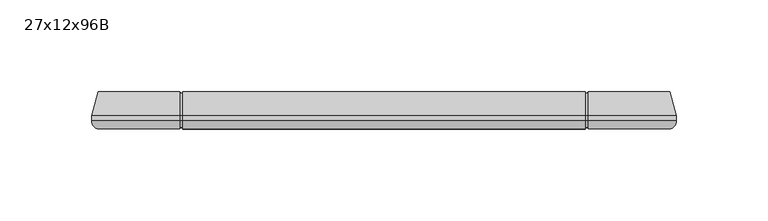
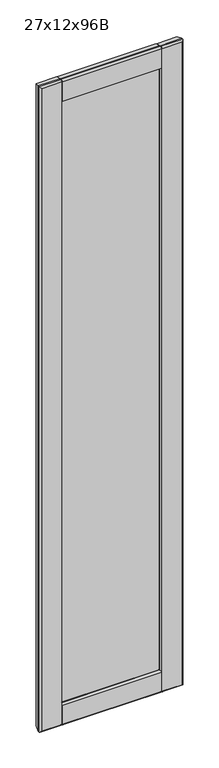
"""IFC4 building model written with IfcOpenShell, lengths in millimetres: furniture geometry, Cabinet-Tall-Merillat-Utility_Double-Marlin : 27x12x96B."""

from ifc_helpers import new_model, si_unit, frame, origin, place, context, project, spatial, polyline, circle_curve, ellipse_curve, outline, extrude, source, transform, mapped, element, save
from ifc_brep_helpers import plane_surface, cylinder_surface, advanced_brep


def furniture_27x12x96b_5ba57cf1(model_context):
    return source(origin(), model_context, "Body", "SolidModel", [
        advanced_brep(
        [(314.6646592, -320.6496, 1651.0), (311.5681667, -325.12, 1647.9035075), (311.5681667, -325.12, 142.7964925), (314.6646592, -320.6496, 139.7), (314.6646592, -317.881, 139.7), (314.6646592, -317.881, 1651.0), (311.1594592, -304.8, 143.2052), (311.1594592, -304.8, 1647.4948), (266.4634964, -304.8, 1602.7988372), (266.4634964, -304.8, 187.9011628), (266.0933647, -305.59375, 188.2712945), (264.0122057, -310.05681, 190.3524535), (264.0122057, -310.05681, 1600.3475465), (266.0933647, -305.59375, 1602.4287055), (265.4119751, -312.2969093, 188.952684), (265.4119751, -312.2969093, 1601.747316), (279.7396592, -312.547, 174.625), (279.7396592, -312.547, 1616.075), (279.7396592, -317.373, 174.625), (279.7396592, -317.373, 1616.075), (265.4119751, -317.6230907, 188.952684), (265.4119751, -317.6230907, 1601.747316), (264.0122057, -319.86319, 190.3524535), (264.0122057, -319.86319, 1600.3475465), (266.0933647, -324.32625, 188.2712945), (266.460629, -325.1138508, 187.9040302), (266.4634964, -325.12, 1602.7988372), (266.0933647, -324.32625, 1602.4287055), (266.460629, -325.12, 142.7964925), (266.460629, -320.6496, 139.7), (-1.3263483, -325.12, 142.7964925), (-4.4228408, -320.6496, 139.7), (43.7413778, -320.6496, 139.7), (43.7413778, -325.12, 142.7964925), (264.873129, -320.6496, 139.7), (264.873129, -325.12, 142.7964925), (45.3288778, -325.12, 142.7964925), (45.3288778, -320.6496, 139.7), (266.460629, -317.881, 139.7), (-4.4228408, -317.881, 139.7), (43.7413778, -317.881, 139.7), (264.873129, -317.881, 139.7), (45.3288778, -317.881, 139.7), (266.460629, -304.8, 143.2052), (-0.9176408, -304.8, 143.2052), (43.7413778, -304.8, 143.2052), (264.873129, -304.8, 143.2052), (45.3288778, -304.8, 143.2052), (46.2296127, -310.05681, 190.3524535), (264.873129, -305.59375, 188.2712945), (264.873129, -304.8, 187.9011628), (45.3288778, -304.8, 187.9011628), (45.3288778, -305.59375, 188.2712945), (44.1484536, -305.59375, 188.2712945), (44.8298432, -312.2969093, 188.952684), (30.5021592, -312.547, 174.625), (30.5021592, -317.373, 174.625), (44.8298432, -317.6230907, 188.952684), (46.2296127, -319.86319, 190.3524535), (44.1484536, -324.32625, 188.2712945), (45.3288778, -324.32625, 188.2712945), (45.3288778, -325.12, 187.9011628), (264.873129, -325.12, 187.9011628), (264.873129, -324.32625, 188.2712945), (-1.3263483, -325.12, 1647.9035075), (-4.4228408, -320.6496, 1651.0), (-4.4228408, -317.881, 1651.0), (-0.9176408, -304.8, 1647.4948), (43.7783219, -304.8, 187.9011628), (43.7783219, -304.8, 1602.7988372), (44.1484536, -305.59375, 1602.4287055), (46.2296127, -310.05681, 1600.3475465), (44.8298432, -312.2969093, 1601.747316), (30.5021592, -312.547, 1616.075), (30.5021592, -317.373, 1616.075), (44.8298432, -317.6230907, 1601.747316), (46.2296127, -319.86319, 1600.3475465), (44.1484536, -324.32625, 1602.4287055), (43.7783219, -325.12, 1602.7988372), (43.7783219, -325.12, 187.9011628), (43.7413778, -325.12, 1647.9035075), (43.7413778, -320.6496, 1651.0), (266.460629, -320.6496, 1651.0), (266.460629, -325.12, 1647.9035075), (45.3288778, -320.6496, 1651.0), (45.3288778, -325.12, 1647.9035075), (264.873129, -325.12, 1647.9035075), (264.873129, -320.6496, 1651.0), (43.7413778, -317.881, 1651.0), (266.460629, -317.881, 1651.0), (45.3288778, -317.881, 1651.0), (264.873129, -317.881, 1651.0), (43.7413778, -304.8, 1647.4948), (266.460629, -304.8, 1647.4948), (45.3288778, -304.8, 1647.4948), (264.873129, -304.8, 1647.4948), (45.3288778, -304.8, 1602.7988372), (264.873129, -304.8, 1602.7988372), (45.3288778, -305.59375, 1602.4287055), (264.873129, -305.59375, 1602.4287055), (264.873129, -324.32625, 1602.4287055), (264.873129, -325.12, 1602.7988372), (45.3288778, -325.12, 1602.7988372), (45.3288778, -324.32625, 1602.4287055), (45.3288778, -305.59375, 1646.8857412), (45.3288778, -317.9855037, 1650.20625), (45.3288778, -320.6496, 1650.20625), (45.3288778, -324.32625, 1647.7526052), (43.7413778, -324.32625, 1602.4287055), (43.7413778, -324.32625, 1647.7526052), (43.7413778, -320.6496, 1650.20625), (43.7413778, -317.9855037, 1650.20625), (43.7413778, -305.59375, 1646.8857412), (43.7413778, -305.59375, 1602.4287055), (266.460629, -305.59375, 1602.4287055), (266.460629, -305.59375, 1646.8857412), (266.460629, -317.9855037, 1650.20625), (266.460629, -320.6496, 1650.20625), (266.460629, -324.32625, 1647.7526052), (266.460629, -324.32625, 1602.4287055), (264.873129, -324.32625, 1647.7526052), (264.873129, -320.6496, 1650.20625), (264.873129, -317.9855037, 1650.20625), (264.873129, -305.59375, 1646.8857412), (266.460629, -324.32625, 188.2712945), (266.460629, -324.32625, 142.9473948), (266.460629, -320.6496, 140.49375), (266.460629, -317.9855037, 140.49375), (266.460629, -305.59375, 143.8142588), (266.460629, -305.59375, 188.2712945), (264.873129, -305.59375, 143.8142588), (264.873129, -317.9855037, 140.49375), (264.873129, -320.6496, 140.49375), (264.873129, -324.32625, 142.9473948), (45.3288778, -324.32625, 142.9473948), (45.3288778, -320.6496, 140.49375), (45.3288778, -317.9855037, 140.49375), (45.3288778, -305.59375, 143.8142588), (43.7413778, -324.32625, 188.2712945), (43.7413778, -305.59375, 188.2712945), (43.7413778, -305.59375, 143.8142588), (43.7413778, -317.9855037, 140.49375), (43.7413778, -320.6496, 140.49375), (43.7413778, -324.32625, 142.9473948)],
        [
            (0, 1, ellipse_curve(frame((309.8894592, -320.6496, 1646.2248), z_axis=(0.7071067811865475, 0.0, -0.7071067811865475), x_axis=(0.7071067811865474, 0.0, 0.7071067811865476)), 6.7531526, 4.7752)),
            (1, 2),
            (2, 3, ellipse_curve(frame((309.8894592, -320.6496, 144.4752), z_axis=(0.7071067811865475, 0.0, 0.7071067811865475), x_axis=(-0.7071067811865474, 0.0, 0.7071067811865476)), 6.7531526, 4.7752)),
            (3, 0),
            (3, 4),
            (4, 5),
            (5, 0),
            (4, 6),
            (6, 7),
            (7, 5),
            (8, 9),
            (9, 10),
            (10, 11),
            (11, 12),
            (12, 13),
            (13, 8),
            (11, 14, ellipse_curve(frame((265.4394592, -310.7223492, 188.9252), z_axis=(0.7071067811865475, 0.0, 0.7071067811865475), x_axis=(-0.7071067811865474, 0.0, 0.7071067811865476)), 2.2271035, 1.5748)),
            (14, 15),
            (15, 12, ellipse_curve(frame((265.4394592, -310.7223492, 1601.7748), z_axis=(0.7071067811865475, 0.0, -0.7071067811865475), x_axis=(0.7071067811865474, 0.0, 0.7071067811865476)), 2.2271035, 1.5748)),
            (14, 16),
            (16, 17),
            (17, 15),
            (16, 18),
            (18, 19),
            (19, 17),
            (18, 20),
            (20, 21),
            (21, 19),
            (20, 22, ellipse_curve(frame((265.4394592, -319.1976508, 188.9252), z_axis=(0.7071067811865475, 0.0, 0.7071067811865475), x_axis=(-0.7071067811865474, 0.0, 0.7071067811865476)), 2.2271035, 1.5748)),
            (22, 23),
            (23, 21, ellipse_curve(frame((265.4394592, -319.1976508, 1601.7748), z_axis=(0.7071067811865475, 0.0, -0.7071067811865475), x_axis=(0.7071067811865474, 0.0, 0.7071067811865476)), 2.2271035, 1.5748)),
            (22, 24),
            (24, 25),
            (25, 26),
            (26, 27),
            (27, 23),
            (2, 28),
            (28, 29, circle_curve(frame((266.460629, -320.6496, 144.4752), z_axis=(1.0, 0.0, 0.0), x_axis=(0.0, 1.0, 0.0)), 4.7752)),
            (29, 3),
            (30, 31, ellipse_curve(frame((0.3523592, -320.6496, 144.4752), z_axis=(0.7071067811865475, 0.0, -0.7071067811865475), x_axis=(0.7071067811865476, 0.0, 0.7071067811865474)), 6.7531526, 4.7752)),
            (31, 32),
            (32, 33, circle_curve(frame((43.7413778, -320.6496, 144.4752), z_axis=(-1.0, 0.0, 0.0), x_axis=(0.0, 1.0, 0.0)), 4.7752)),
            (33, 30),
            (34, 35, circle_curve(frame((264.873129, -320.6496, 144.4752), z_axis=(-1.0, 0.0, 0.0), x_axis=(0.0, 1.0, 0.0)), 4.7752)),
            (35, 36),
            (36, 37, circle_curve(frame((45.3288778, -320.6496, 144.4752), z_axis=(1.0, 0.0, 0.0), x_axis=(0.0, 1.0, 0.0)), 4.7752)),
            (37, 34),
            (29, 38),
            (38, 4),
            (31, 39),
            (39, 40),
            (40, 32),
            (41, 34),
            (37, 42),
            (42, 41),
            (38, 43),
            (43, 6),
            (39, 44),
            (44, 45),
            (45, 40),
            (46, 41),
            (42, 47),
            (47, 46),
            (48, 11),
            (10, 49),
            (49, 50),
            (50, 51),
            (51, 52),
            (52, 53),
            (53, 48),
            (48, 54, ellipse_curve(frame((44.8023592, -310.7223492, 188.9252), z_axis=(0.7071067811865475, 0.0, -0.7071067811865475), x_axis=(0.7071067811865476, 0.0, 0.7071067811865474)), 2.2271035, 1.5748)),
            (54, 14),
            (54, 55),
            (55, 16),
            (55, 56),
            (56, 18),
            (56, 57),
            (57, 20),
            (57, 58, ellipse_curve(frame((44.8023592, -319.1976508, 188.9252), z_axis=(0.7071067811865475, 0.0, -0.7071067811865475), x_axis=(0.7071067811865476, 0.0, 0.7071067811865474)), 2.2271035, 1.5748)),
            (58, 22),
            (58, 59),
            (59, 60),
            (60, 61),
            (61, 62),
            (62, 63),
            (63, 24),
            (30, 64),
            (64, 65, ellipse_curve(frame((0.3523592, -320.6496, 1646.2248), z_axis=(-0.7071067811865475, 0.0, -0.7071067811865475), x_axis=(0.7071067811865474, 0.0, -0.7071067811865476)), 6.7531526, 4.7752)),
            (65, 31),
            (65, 66),
            (66, 39),
            (66, 67),
            (67, 44),
            (68, 69),
            (69, 70),
            (70, 71),
            (71, 48),
            (53, 68),
            (71, 72, ellipse_curve(frame((44.8023592, -310.7223492, 1601.7748), z_axis=(-0.7071067811865475, 0.0, -0.7071067811865475), x_axis=(0.7071067811865474, 0.0, -0.7071067811865476)), 2.2271035, 1.5748)),
            (72, 54),
            (72, 73),
            (73, 55),
            (73, 74),
            (74, 56),
            (74, 75),
            (75, 57),
            (75, 76, ellipse_curve(frame((44.8023592, -319.1976508, 1601.7748), z_axis=(-0.7071067811865475, 0.0, -0.7071067811865475), x_axis=(0.7071067811865474, 0.0, -0.7071067811865476)), 2.2271035, 1.5748)),
            (76, 58),
            (76, 77),
            (77, 78),
            (78, 79),
            (79, 59),
            (64, 80),
            (80, 81, circle_curve(frame((43.7413778, -320.6496, 1646.2248), z_axis=(-1.0, 0.0, 0.0), x_axis=(0.0, 1.0, 0.0)), 4.7752)),
            (81, 65),
            (0, 82),
            (82, 83, circle_curve(frame((266.460629, -320.6496, 1646.2248), z_axis=(1.0, 0.0, 0.0), x_axis=(0.0, 1.0, 0.0)), 4.7752)),
            (83, 1),
            (84, 85, circle_curve(frame((45.3288778, -320.6496, 1646.2248), z_axis=(1.0, 0.0, 0.0), x_axis=(0.0, 1.0, 0.0)), 4.7752)),
            (85, 86),
            (86, 87, circle_curve(frame((264.873129, -320.6496, 1646.2248), z_axis=(-1.0, 0.0, 0.0), x_axis=(0.0, 1.0, 0.0)), 4.7752)),
            (87, 84),
            (81, 88),
            (88, 66),
            (5, 89),
            (89, 82),
            (90, 84),
            (87, 91),
            (91, 90),
            (88, 92),
            (92, 67),
            (7, 93),
            (93, 89),
            (94, 90),
            (91, 95),
            (95, 94),
            (43, 9),
            (8, 93),
            (92, 69),
            (68, 45),
            (96, 94),
            (95, 97),
            (97, 96),
            (50, 46),
            (47, 51),
            (12, 71),
            (70, 98),
            (98, 96),
            (97, 99),
            (99, 13),
            (15, 72),
            (17, 73),
            (19, 74),
            (21, 75),
            (23, 76),
            (27, 100),
            (100, 101),
            (101, 102),
            (102, 103),
            (103, 77),
            (83, 26),
            (25, 28),
            (33, 79),
            (78, 80),
            (85, 102),
            (101, 86),
            (35, 62),
            (61, 36),
            (98, 104),
            (104, 105),
            (105, 106),
            (106, 107, circle_curve(frame((45.3288778, -320.6496, 1646.2248), z_axis=(1.0, 0.0, 0.0), x_axis=(0.0, 0.0, 1.0)), 3.98145)),
            (107, 103),
            (78, 108),
            (108, 109),
            (109, 110, circle_curve(frame((43.7413778, -320.6496, 1646.2248), z_axis=(-1.0, 0.0, 0.0), x_axis=(0.0, 0.0, 1.0)), 3.98145)),
            (110, 111),
            (111, 112),
            (112, 113),
            (113, 69),
            (77, 108),
            (107, 109),
            (106, 110),
            (105, 111),
            (104, 112),
            (70, 113),
            (8, 114),
            (114, 115),
            (115, 116),
            (116, 117),
            (117, 118, circle_curve(frame((266.460629, -320.6496, 1646.2248), z_axis=(1.0, 0.0, 0.0), x_axis=(0.0, 0.0, 1.0)), 3.98145)),
            (118, 119),
            (119, 26),
            (100, 120),
            (120, 121, circle_curve(frame((264.873129, -320.6496, 1646.2248), z_axis=(-1.0, 0.0, 0.0), x_axis=(0.0, 0.0, 1.0)), 3.98145)),
            (121, 122),
            (122, 123),
            (123, 99),
            (119, 27),
            (118, 120),
            (117, 121),
            (116, 122),
            (115, 123),
            (114, 13),
            (25, 124),
            (124, 125),
            (125, 126, circle_curve(frame((266.460629, -320.6496, 144.4752), z_axis=(1.0, 0.0, 0.0), x_axis=(0.0, 0.0, 1.0)), 3.98145)),
            (126, 127),
            (127, 128),
            (128, 129),
            (129, 9),
            (49, 130),
            (130, 131),
            (131, 132),
            (132, 133, circle_curve(frame((264.873129, -320.6496, 144.4752), z_axis=(-1.0, 0.0, 0.0), x_axis=(0.0, 0.0, 1.0)), 3.98145)),
            (133, 63),
            (129, 10),
            (128, 130),
            (127, 131),
            (126, 132),
            (125, 133),
            (124, 24),
            (60, 134),
            (134, 135, circle_curve(frame((45.3288778, -320.6496, 144.4752), z_axis=(1.0, 0.0, 0.0), x_axis=(0.0, 0.0, 1.0)), 3.98145)),
            (135, 136),
            (136, 137),
            (137, 52),
            (138, 79),
            (68, 139),
            (139, 140),
            (140, 141),
            (141, 142),
            (142, 143, circle_curve(frame((43.7413778, -320.6496, 144.4752), z_axis=(-1.0, 0.0, 0.0), x_axis=(0.0, 0.0, 1.0)), 3.98145)),
            (143, 138),
            (138, 59),
            (53, 139),
            (137, 140),
            (136, 141),
            (135, 142),
            (134, 143),
        ],
        [
            cylinder_surface(frame((309.8894592, -320.6496, 1651.0), z_axis=(0.0, 0.0, 1.0), x_axis=(0.0, 1.0, 0.0)), 4.7752),
            plane_surface(frame((314.6646592, -320.6496, 1651.0), z_axis=(1.0, 0.0, 0.0), x_axis=(0.0, 0.0, -1.0))),
            plane_surface(frame((314.6646592, -317.881, 1651.0), z_axis=(0.9659229350723619, 0.25882983502910506, 0.0), x_axis=(0.0, 0.0, -1.0))),
            plane_surface(frame((266.4634964, -304.8, 1602.7988372), z_axis=(-0.9063077870366099, 0.4226182617407856, 0.0), x_axis=(0.0, 0.0, -1.0))),
            cylinder_surface(frame((265.4394592, -310.7223492, 1651.0), z_axis=(0.0, 0.0, 1.0000000000000002), x_axis=(-0.01745240643729364, -0.9998476951563912, 0.0)), 1.5748),
            plane_surface(frame((265.4119751, -312.2969093, 1601.747316), z_axis=(-0.017452406437322144, -0.9998476951563906, 0.0), x_axis=(0.0, 0.0, -1.0))),
            plane_surface(frame((279.7396592, -312.547, 1616.075), z_axis=(-1.0, 0.0, 0.0), x_axis=(0.0, 0.0, -1.0))),
            plane_surface(frame((279.7396592, -317.373, 1616.075), z_axis=(-0.01745240643727848, 0.9998476951563914, 0.0), x_axis=(0.0, 0.0, -1.0))),
            cylinder_surface(frame((265.4394592, -319.1976508, 1651.0), z_axis=(0.0, 0.0, 1.0000000000000002), x_axis=(-0.9063077870367326, -0.42261826174052236, 0.0)), 1.5748),
            plane_surface(frame((264.0122057, -319.86319, 1600.3475465), z_axis=(-0.9063077870366333, -0.4226182617407352, 0.0), x_axis=(0.0, 0.0, -1.0))),
            cylinder_surface(frame((314.6646592, -320.6496, 144.4752), z_axis=(1.0, 0.0, 0.0), x_axis=(0.0, 1.0, 0.0)), 4.7752),
            plane_surface(frame((314.6646592, -320.6496, 139.7), z_axis=(0.0, 0.0, -1.0), x_axis=(-1.0, 0.0, 0.0))),
            plane_surface(frame((314.6646592, -317.881, 139.7), z_axis=(0.0, 0.25882983502910506, -0.9659229350723619), x_axis=(-1.0, 0.0, 0.0))),
            plane_surface(frame((266.4634964, -304.8, 187.9011628), z_axis=(0.0, 0.4226182617407856, 0.9063077870366099), x_axis=(-1.0, 0.0, 0.0))),
            cylinder_surface(frame((314.6646592, -310.7223492, 188.9252), z_axis=(1.0000000000000002, 0.0, 0.0), x_axis=(0.0, -0.9998476951563912, 0.01745240643729364)), 1.5748),
            plane_surface(frame((265.4119751, -312.2969093, 188.952684), z_axis=(0.0, -0.9998476951563906, 0.017452406437322144), x_axis=(-1.0, 0.0, 0.0))),
            plane_surface(frame((279.7396592, -312.547, 174.625), z_axis=(0.0, 0.0, 1.0), x_axis=(-1.0, 0.0, 0.0))),
            plane_surface(frame((279.7396592, -317.373, 174.625), z_axis=(0.0, 0.9998476951563914, 0.01745240643727848), x_axis=(-1.0, 0.0, 0.0))),
            cylinder_surface(frame((314.6646592, -319.1976508, 188.9252), z_axis=(1.0000000000000002, 0.0, 0.0), x_axis=(0.0, -0.42261826174052236, 0.9063077870367326)), 1.5748),
            plane_surface(frame((264.0122057, -319.86319, 190.3524535), z_axis=(0.0, -0.4226182617407352, 0.9063077870366333), x_axis=(-1.0, 0.0, 0.0))),
            cylinder_surface(frame((0.3523592, -320.6496, 139.7), z_axis=(0.0, 0.0, -1.0), x_axis=(0.0, 1.0, 0.0)), 4.7752),
            plane_surface(frame((-4.4228408, -320.6496, 139.7), z_axis=(-1.0, 0.0, 0.0), x_axis=(0.0, 0.0, 1.0))),
            plane_surface(frame((-4.4228408, -317.881, 139.7), z_axis=(-0.9659229350723619, 0.25882983502910506, 0.0), x_axis=(0.0, 0.0, 1.0))),
            plane_surface(frame((43.7783219, -304.8, 187.9011628), z_axis=(0.9063077870366099, 0.4226182617407856, 0.0), x_axis=(0.0, 0.0, 1.0))),
            cylinder_surface(frame((44.8023592, -310.7223492, 139.7), z_axis=(0.0, 0.0, -1.0000000000000002), x_axis=(0.01745240643729364, -0.9998476951563912, 0.0)), 1.5748),
            plane_surface(frame((44.8298432, -312.2969093, 188.952684), z_axis=(0.017452406437322144, -0.9998476951563906, 0.0), x_axis=(0.0, 0.0, 1.0))),
            plane_surface(frame((30.5021592, -312.547, 174.625), z_axis=(1.0, 0.0, 0.0), x_axis=(0.0, 0.0, 1.0))),
            plane_surface(frame((30.5021592, -317.373, 174.625), z_axis=(0.01745240643727848, 0.9998476951563914, 0.0), x_axis=(0.0, 0.0, 1.0))),
            cylinder_surface(frame((44.8023592, -319.1976508, 139.7), z_axis=(0.0, 0.0, -1.0000000000000002), x_axis=(0.9063077870367326, -0.42261826174052236, 0.0)), 1.5748),
            plane_surface(frame((46.2296127, -319.86319, 190.3524535), z_axis=(0.9063077870366333, -0.4226182617407352, 0.0), x_axis=(0.0, 0.0, 1.0))),
            cylinder_surface(frame((-4.4228408, -320.6496, 1646.2248), z_axis=(-1.0, 0.0, 0.0), x_axis=(0.0, 1.0, 0.0)), 4.7752),
            plane_surface(frame((-4.4228408, -320.6496, 1651.0), z_axis=(0.0, 0.0, 1.0), x_axis=(1.0, 0.0, 0.0))),
            plane_surface(frame((-4.4228408, -317.881, 1651.0), z_axis=(0.0, 0.25882983502910506, 0.9659229350723619), x_axis=(1.0, 0.0, 0.0))),
            plane_surface(frame((-0.9176408, -304.8, 1647.4948), z_axis=(0.0, 1.0, 0.0), x_axis=(1.0, 0.0, 0.0))),
            plane_surface(frame((43.7783219, -304.8, 1602.7988372), z_axis=(0.0, 0.4226182617407856, -0.9063077870366099), x_axis=(1.0, 0.0, 0.0))),
            cylinder_surface(frame((-4.4228408, -310.7223492, 1601.7748), z_axis=(-1.0000000000000002, 0.0, 0.0), x_axis=(0.0, -0.9998476951563912, -0.01745240643729364)), 1.5748),
            plane_surface(frame((44.8298432, -312.2969093, 1601.747316), z_axis=(0.0, -0.9998476951563906, -0.017452406437322144), x_axis=(1.0, 0.0, 0.0))),
            plane_surface(frame((30.5021592, -312.547, 1616.075), z_axis=(0.0, 0.0, -1.0), x_axis=(1.0, 0.0, 0.0))),
            plane_surface(frame((30.5021592, -317.373, 1616.075), z_axis=(0.0, 0.9998476951563914, -0.01745240643727848), x_axis=(1.0, 0.0, 0.0))),
            cylinder_surface(frame((-4.4228408, -319.1976508, 1601.7748), z_axis=(-1.0000000000000002, 0.0, 0.0), x_axis=(0.0, -0.42261826174052236, -0.9063077870367326)), 1.5748),
            plane_surface(frame((46.2296127, -319.86319, 1600.3475465), z_axis=(0.0, -0.4226182617407352, -0.9063077870366333), x_axis=(1.0, 0.0, 0.0))),
            plane_surface(frame((43.7783219, -325.12, 1602.7988372), z_axis=(0.0, -1.0, 0.0), x_axis=(1.0, 0.0, 0.0))),
            plane_surface(frame((45.3288778, -325.12, 1602.7988372), z_axis=(-1.0, 0.0, 0.0), x_axis=(0.0, 0.9063077870366174, -0.42261826174076933))),
            plane_surface(frame((43.7413778, -325.12, 1602.7988372), z_axis=(1.0, 0.0, 0.0), x_axis=(0.0, -0.9063077870366174, 0.42261826174076933))),
            plane_surface(frame((45.3288778, -325.12, 1602.7988372), z_axis=(0.0, 0.42261826174076933, 0.9063077870366174), x_axis=(-1.0, 0.0, 0.0))),
            plane_surface(frame((45.3288778, -324.32625, 1602.4287055), z_axis=(0.0, -1.0, 0.0), x_axis=(-1.0, 0.0, 0.0))),
            cylinder_surface(frame((43.7413778, -320.6496, 1646.2248), z_axis=(-1.0, 0.0, 0.0), x_axis=(0.0, 0.0, 1.0)), 3.98145),
            plane_surface(frame((45.3288778, -320.6496, 1650.20625), z_axis=(0.0, 0.0, 1.0), x_axis=(-1.0, 0.0, 0.0))),
            plane_surface(frame((45.3288778, -317.9855037, 1650.20625), z_axis=(0.0, 0.258829835029167, 0.9659229350723454), x_axis=(-1.0, 0.0, 0.0))),
            plane_surface(frame((45.3288778, -305.59375, 1646.8857412), z_axis=(0.0, 1.0, 0.0), x_axis=(-1.0, 0.0, 0.0))),
            plane_surface(frame((45.3288778, -305.59375, 1602.4287055), z_axis=(0.0, -0.422618261740684, 0.9063077870366572), x_axis=(-1.0, 0.0, 0.0))),
            plane_surface(frame((266.460629, -325.12, 1602.7988372), z_axis=(-1.0, 0.0, 0.0), x_axis=(0.0, 0.9063077870366261, -0.42261826174075084))),
            plane_surface(frame((264.873129, -325.12, 1602.7988372), z_axis=(1.0, 0.0, 0.0), x_axis=(0.0, -0.9063077870366261, 0.42261826174075084))),
            plane_surface(frame((266.460629, -325.12, 1602.7988372), z_axis=(0.0, 0.42261826174075084, 0.9063077870366261), x_axis=(-1.0, 0.0, 0.0))),
            plane_surface(frame((266.460629, -324.32625, 1602.4287055), z_axis=(0.0, -1.0, 0.0), x_axis=(-1.0, 0.0, 0.0))),
            cylinder_surface(frame((264.873129, -320.6496, 1646.2248), z_axis=(-1.0, 0.0, 0.0), x_axis=(0.0, 0.0, 1.0)), 3.98145),
            plane_surface(frame((266.460629, -320.6496, 1650.20625), z_axis=(0.0, 0.0, 1.0), x_axis=(-1.0, 0.0, 0.0))),
            plane_surface(frame((266.460629, -317.9855037, 1650.20625), z_axis=(0.0, 0.25882983502917056, 0.9659229350723444), x_axis=(-1.0, 0.0, 0.0))),
            plane_surface(frame((266.460629, -305.59375, 1646.8857412), z_axis=(0.0, 1.0, 0.0), x_axis=(-1.0, 0.0, 0.0))),
            plane_surface(frame((266.460629, -305.59375, 1602.4287055), z_axis=(0.0, -0.422618261740703, 0.9063077870366484), x_axis=(-1.0, 0.0, 0.0))),
            plane_surface(frame((266.460629, -320.6496, 149.2504), z_axis=(-1.0, 0.0, 0.0), x_axis=(0.0, -1.0, 0.0))),
            plane_surface(frame((264.873129, -320.6496, 149.2504), z_axis=(1.0, 0.0, 0.0), x_axis=(0.0, 1.0, 0.0))),
            plane_surface(frame((266.460629, -304.8, 187.9011628), z_axis=(0.0, -0.42261826174076006, -0.9063077870366217), x_axis=(-1.0, 0.0, 0.0))),
            plane_surface(frame((266.460629, -305.59375, 188.2712945), z_axis=(0.0, 1.0, 0.0), x_axis=(-1.0, 0.0, 0.0))),
            plane_surface(frame((266.460629, -305.59375, 143.8142588), z_axis=(0.0, 0.2588298350294429, -0.9659229350722714), x_axis=(-1.0, 0.0, 0.0))),
            plane_surface(frame((266.460629, -317.9855037, 140.49375), z_axis=(0.0, 0.0, -1.0), x_axis=(-1.0, 0.0, 0.0))),
            cylinder_surface(frame((264.873129, -320.6496, 144.4752), z_axis=(-1.0, 0.0, 0.0), x_axis=(0.0, 0.0, 1.0)), 3.98145),
            plane_surface(frame((266.460629, -324.32625, 142.9473948), z_axis=(0.0, -1.0, 0.0), x_axis=(-1.0, 0.0, 0.0))),
            plane_surface(frame((266.460629, -324.32625, 188.2712945), z_axis=(0.0, 0.4226182617407291, -0.9063077870366362), x_axis=(-1.0, 0.0, 0.0))),
            plane_surface(frame((45.3288778, -324.32625, 188.2712945), z_axis=(-1.0, 0.0, 0.0), x_axis=(0.0, -0.9063077870366145, -0.42261826174077555))),
            plane_surface(frame((43.7413778, -324.32625, 188.2712945), z_axis=(1.0, 0.0, 0.0), x_axis=(0.0, 0.9063077870366145, 0.42261826174077555))),
            plane_surface(frame((45.3288778, -324.32625, 188.2712945), z_axis=(0.0, 0.42261826174077555, -0.9063077870366145), x_axis=(-1.0, 0.0, 0.0))),
            plane_surface(frame((45.3288778, -304.8, 187.9011628), z_axis=(0.0, -0.4226182617407416, -0.9063077870366304), x_axis=(-1.0, 0.0, 0.0))),
            plane_surface(frame((45.3288778, -305.59375, 188.2712945), z_axis=(0.0, 1.0, 0.0), x_axis=(-1.0, 0.0, 0.0))),
            plane_surface(frame((45.3288778, -305.59375, 143.8142588), z_axis=(0.0, 0.2588298350294438, -0.9659229350722711), x_axis=(-1.0, 0.0, 0.0))),
            plane_surface(frame((45.3288778, -317.9855037, 140.49375), z_axis=(0.0, 0.0, -1.0), x_axis=(-1.0, 0.0, 0.0))),
            cylinder_surface(frame((43.7413778, -320.6496, 144.4752), z_axis=(-1.0, 0.0, 0.0), x_axis=(0.0, 0.0, 1.0)), 3.98145),
            plane_surface(frame((45.3288778, -324.32625, 142.9473948), z_axis=(0.0, -1.0, 0.0), x_axis=(-1.0, 0.0, 0.0))),
        ],
        [
            (0, [[1, 2, 3, 4]]),
            (1, [[-4, 5, 6, 7]]),
            (2, [[-6, 8, 9, 10]]),
            (3, [[11, 12, 13, 14, 15, 16]]),
            (4, [[-14, 17, 18, 19]]),
            (5, [[-18, 20, 21, 22]]),
            (6, [[-21, 23, 24, 25]]),
            (7, [[-24, 26, 27, 28]]),
            (8, [[-27, 29, 30, 31]]),
            (9, [[-30, 32, 33, 34, 35, 36]]),
            (10, [[-3, 37, 38, 39]]),
            (10, [[40, 41, 42, 43]]),
            (10, [[44, 45, 46, 47]]),
            (11, [[-5, -39, 48, 49]]),
            (11, [[50, 51, 52, -41]]),
            (11, [[53, -47, 54, 55]]),
            (12, [[-8, -49, 56, 57]]),
            (12, [[58, 59, 60, -51]]),
            (12, [[61, -55, 62, 63]]),
            (13, [[64, -13, 65, 66, 67, 68, 69, 70]]),
            (14, [[-17, -64, 71, 72]]),
            (15, [[-20, -72, 73, 74]]),
            (16, [[-23, -74, 75, 76]]),
            (17, [[-26, -76, 77, 78]]),
            (18, [[-29, -78, 79, 80]]),
            (19, [[-80, 81, 82, 83, 84, 85, 86, -32]]),
            (20, [[-40, 87, 88, 89]]),
            (21, [[-50, -89, 90, 91]]),
            (22, [[-58, -91, 92, 93]]),
            (23, [[94, 95, 96, 97, -70, 98]]),
            (24, [[-71, -97, 99, 100]]),
            (25, [[-73, -100, 101, 102]]),
            (26, [[-75, -102, 103, 104]]),
            (27, [[-77, -104, 105, 106]]),
            (28, [[-79, -106, 107, 108]]),
            (29, [[-108, 109, 110, 111, 112, -81]]),
            (30, [[-88, 113, 114, 115]]),
            (30, [[-1, 116, 117, 118]]),
            (30, [[119, 120, 121, 122]]),
            (31, [[-90, -115, 123, 124]]),
            (31, [[-7, 125, 126, -116]]),
            (31, [[127, -122, 128, 129]]),
            (32, [[-92, -124, 130, 131]]),
            (32, [[-10, 132, 133, -125]]),
            (32, [[134, -129, 135, 136]]),
            (33, [[-9, -57, 137, -11, 138, -132]]),
            (33, [[-93, -131, 139, -94, 140, -59]]),
            (33, [[141, -136, 142, 143]]),
            (33, [[144, -63, 145, -67]]),
            (34, [[146, -96, 147, 148, -143, 149, 150, -15]]),
            (35, [[-19, 151, -99, -146]]),
            (36, [[-22, 152, -101, -151]]),
            (37, [[-25, 153, -103, -152]]),
            (38, [[-28, 154, -105, -153]]),
            (39, [[-31, 155, -107, -154]]),
            (40, [[-155, -36, 156, 157, 158, 159, 160, -109]]),
            (41, [[-2, -118, 161, -34, 162, -37]]),
            (41, [[-87, -43, 163, -111, 164, -113]]),
            (41, [[165, -158, 166, -120]]),
            (41, [[167, -84, 168, -45]]),
            (42, [[169, 170, 171, 172, 173, -159, -165, -119, -127, -134, -141, -148]]),
            (43, [[174, 175, 176, 177, 178, 179, 180, -139, -130, -123, -114, -164]]),
            (44, [[-174, -110, 181]]),
            (45, [[-173, 182, -175, -181, -160]]),
            (46, [[-172, 183, -176, -182]]),
            (47, [[-171, 184, -177, -183]]),
            (48, [[-170, 185, -178, -184]]),
            (49, [[-169, -147, 186, -179, -185]]),
            (50, [[-180, -186, -95]]),
            (51, [[187, 188, 189, 190, 191, 192, 193, -161, -117, -126, -133, -138]]),
            (52, [[194, 195, 196, 197, 198, -149, -142, -135, -128, -121, -166, -157]]),
            (53, [[-193, 199, -35]]),
            (54, [[-192, 200, -194, -156, -199]]),
            (55, [[-191, 201, -195, -200]]),
            (56, [[-190, 202, -196, -201]]),
            (57, [[-189, 203, -197, -202]]),
            (58, [[-188, 204, -150, -198, -203]]),
            (59, [[-187, -16, -204]]),
            (60, [[205, 206, 207, 208, 209, 210, 211, -137, -56, -48, -38, -162]]),
            (61, [[212, 213, 214, 215, 216, -85, -167, -44, -53, -61, -144, -66]]),
            (62, [[-211, 217, -12]]),
            (63, [[-210, 218, -212, -65, -217]]),
            (64, [[-209, 219, -213, -218]]),
            (65, [[-208, 220, -214, -219]]),
            (66, [[-207, 221, -215, -220]]),
            (67, [[-206, 222, -86, -216, -221]]),
            (68, [[-205, -33, -222]]),
            (69, [[223, 224, 225, 226, 227, -68, -145, -62, -54, -46, -168, -83]]),
            (70, [[228, -163, -42, -52, -60, -140, 229, 230, 231, 232, 233, 234]]),
            (71, [[-228, 235, -112]]),
            (72, [[-229, -98, 236]]),
            (73, [[-227, 237, -230, -236, -69]]),
            (74, [[-226, 238, -231, -237]]),
            (75, [[-225, 239, -232, -238]]),
            (76, [[-224, 240, -233, -239]]),
            (77, [[-223, -82, -235, -234, -240]]),
        ],
    ),
        extrude(outline(polyline([(30.5021592, -317.373), (30.5021592, -312.547), (279.7396592, -312.547), (279.7396592, -317.373), (30.5021592, -317.373)])), frame((0.0, 0.0, 174.625), z_axis=(0.0, 0.0, 1.0), x_axis=(1.0, 0.0, 0.0)), (0.0, 0.0, 1.0), 1441.45),
    ])


if __name__ == "__main__":
    model = new_model("IFC4")
    model_context = context("Model", 3, world=origin())
    ifc_project = project(units=[si_unit("LENGTHUNIT", "METRE", prefix="MILLI")], contexts=[model_context])
    site = spatial("IfcSite", under=ifc_project)
    building = spatial("IfcBuilding", under=site)
    placement = place(None, origin())
    furniture_27x12x96b_shape = furniture_27x12x96b_5ba57cf1(model_context)
    element("IfcFurniture", 1, ObjectType="Cabinet-Tall-Merillat-Utility_Double-Marlin : 27x12x96B", at=placement, inside=building, context=model_context, shape_type="MappedRepresentation", body=[
        mapped(furniture_27x12x96b_shape, transform((0.0, 0.0, 0.0), x_axis=(1.0, 0.0, 0.0), y_axis=(0.0, 1.0, 0.0), z_axis=(0.0, 0.0, 1.0))),
    ])
    save(model, "model.ifc")

# Revit data of these elements
# Type "Cabinet-Tall-Merillat-Utility_Double-Marlin : 27x12x96B"
#   URL = "http://www.merillat.com/"
#   Toe Kick Note = "Toe Kick Covering is not included. To be purchased Separately. \r\n\r\n Toe Kick Covering is not included. To be purchased Separately."
#   Product Page URL = "http://www.merillat.com/our-products/rooms/kitchen/"
#   Product Line = "Express"
#   Product Group = "Tall Cabinet"
#   Product Documentation Link = "http://merillatbusiness.com/wp-content/uploads/2014/07/Merillat_Classic_Catalog.pdf"
#   Model = "U3096B"
#   Manufacturer = "Merillat"
#   Finish = "Wood"
#   Description = "Tall Utility Cabinet Double"
#   Construction Type = "Tall Cabinet"
#   Cabinet Construction Note = ""
#   Assembly Code = "C1030410"
#   Spacing = 0' - 1"
#   Door Spacing = 0' - 0 1/8"
#   Cabinet Upper Door Height = 2' - 5"
#   Cabinet Door Width = 1' - 0 9/16"
#   Cabinet Door Height = 4' - 11 1/2"
#   Depth = 1' - 0"
#   Height = 8' - 0"
#   Toe Depth = 0' - 2 25/32"
#   Toe Height = 0' - 4 1/2"
#   Width = 2' - 3"
#   COBie.Type = no
#   Partial Overlay Butt = yes
#   Partial Overlay = no
#   Full Overlay Butt = no
#   Full Overlay = no
#   Elevation Swing Line = yes
#   Toe Kick Material = Wood - Merillat - Raw Particle Board
#   Door Drawer Material = Wood - Merillat - Pecan(1)
#   Cabinet Material = Wood - Merillat - Pecan(1)
#   Cabinet Door Style = element 776454
# Element 1 (IfcFurniture, "Cabinet-Tall-Merillat-Utility_Double-Marlin : 27x12x96B")
#   Materials on its faces: "Wood - Merillat - Pecan(1)", "Wood - Merillat - Raw Particle Board"
# Materials
#   "Wood - Merillat - Raw Particle Board": class "Plastic", colour RGB 80 80 80, transparency 0, Description = "Plastic Laminate - Navy", Cost = 0
#   "Wood - Merillat - Pecan(1)": class "Wood", colour RGB 108 67 43, transparency 0, Cost = 0
